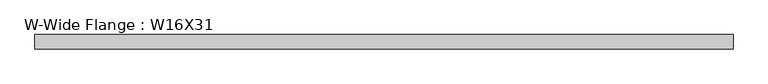
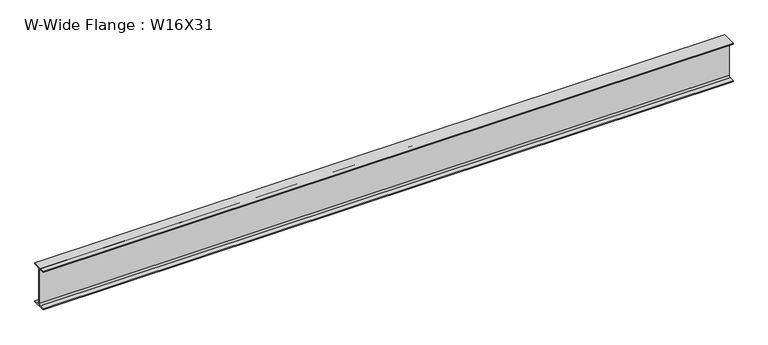
"""IFC4 building model written with IfcOpenShell, lengths in millimetres: beam geometry, W-Wide Flange : W16X31."""

from ifc_helpers import new_model, si_unit, point, frame, frame_2d, origin, place, context, project, spatial, polyline, circle_curve, trimmed, segment, composite_curve, outline, extrude, source, transform, mapped, element, save


def w_wide_flange_w16x31_34482971(model_context):
    return source(origin(), model_context, "Body", "SweptSolid", [
        extrude(outline(composite_curve([segment(polyline([(70.231, -190.754), (70.231, -201.93), (-70.231, -201.93), (-70.231, -190.754), (-20.8915, -190.754)]), True, "CONTINUOUS"), segment(trimmed(circle_curve(frame_2d((-20.8915, -173.355)), 17.399), [point((-20.8915, -190.754))], [point((-3.4925, -173.355))], True, "CARTESIAN"), True, "CONTINUOUS"), segment(polyline([(-3.4925, -173.355), (-3.4925, 173.355)]), True, "CONTINUOUS"), segment(trimmed(circle_curve(frame_2d((-20.8915, 173.355)), 17.399), [point((-3.4925, 173.355))], [point((-20.8915, 190.754))], True, "CARTESIAN"), True, "CONTINUOUS"), segment(polyline([(-20.8915, 190.754), (-70.231, 190.754), (-70.231, 201.93), (70.231, 201.93), (70.231, 190.754), (20.8915, 190.754)]), True, "CONTINUOUS"), segment(trimmed(circle_curve(frame_2d((20.8915, 173.355)), 17.399), [point((20.8915, 190.754))], [point((3.4925, 173.355))], True, "CARTESIAN"), True, "CONTINUOUS"), segment(polyline([(3.4925, 173.355), (3.4925, -173.355)]), True, "CONTINUOUS"), segment(trimmed(circle_curve(frame_2d((20.8915, -173.355)), 17.399), [point((3.4925, -173.355))], [point((20.8915, -190.754))], True, "CARTESIAN"), True, "CONTINUOUS"), segment(polyline([(20.8915, -190.754), (70.231, -190.754)]), True, "CONTINUOUS")], self_intersect=False)), frame((-3413.0955194, 0.0, 0.0), z_axis=(1.0, 0.0, 0.0), x_axis=(0.0, 1.0, 0.0)), (0.0, 0.0, 1.0), 6793.3379351),
    ])


if __name__ == "__main__":
    model = new_model("IFC4")
    model_context = context("Model", 3, world=origin())
    ifc_project = project(units=[si_unit("LENGTHUNIT", "METRE", prefix="MILLI")], contexts=[model_context])
    site = spatial("IfcSite", under=ifc_project)
    building = spatial("IfcBuilding", under=site)
    placement = place(None, origin())
    w_wide_flange_w16x31_shape = w_wide_flange_w16x31_34482971(model_context)
    element("IfcBeam", 1, ObjectType="W-Wide Flange : W16X31", at=placement, inside=building, context=model_context, shape_type="MappedRepresentation", body=[
        mapped(w_wide_flange_w16x31_shape, transform((0.0, 0.0, 0.0), x_axis=(1.0, 0.0, 0.0), y_axis=(0.0, 1.0, 0.0), z_axis=(0.0, 0.0, 1.0))),
    ])
    save(model, "model.ifc")

# Revit data of these elements
# Type "W-Wide Flange : W16X31"
#   Assembly Code = "B10"
#   W = 31
#   Start Extension Calculation [instance default] = 10' - 0"
#   Start Extension [instance default] = -0' - 0 1/2"
#   End Extension Calculation [instance default] = 10' - 0"
#   End Extension [instance default] = -0' - 0 1/2"
#   Length [instance default] = 5' - 0"
#   bf = 0' - 5.53"
#   d = 1' - 3.9"
#   k = 0' - 1 1/8"
#   k2 = 0' - 0.685"
#   tf = 0' - 0.44"
#   tw = 0' - 0.275"
#   A = 0.0634028 SF
#   Beam Material [instance default] = Metal - Steel - ASTM A992
# Element 1 (IfcBeam, "W-Wide Flange : W16X31")
#   Materials on its faces: "Metal - Steel - ASTM A992"
# Materials
#   "Metal - Steel - ASTM A992": class "Metal", colour RGB 128 0 0, transparency 0
